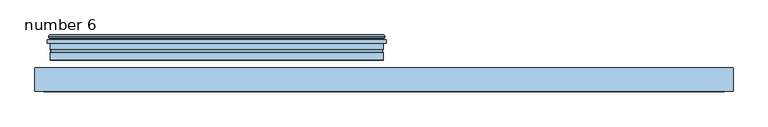
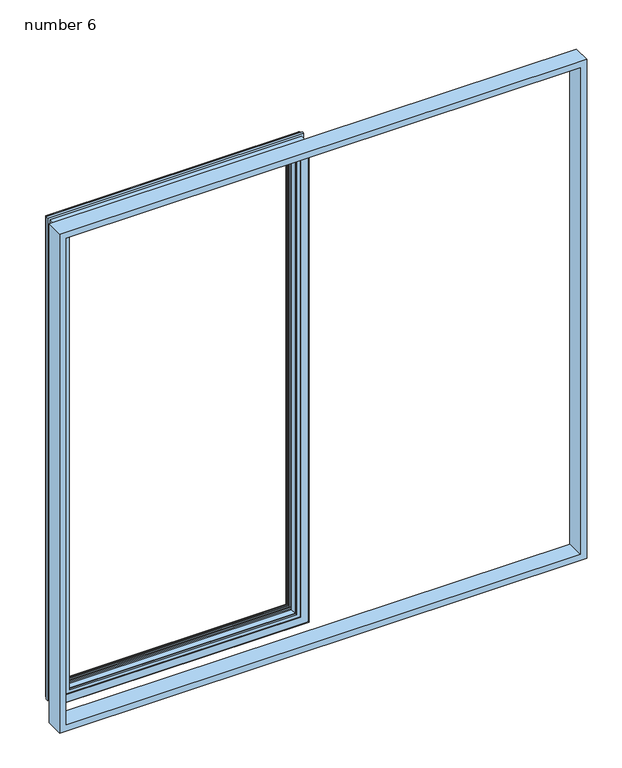
"""IFC4 building model written with IfcOpenShell, lengths in millimetres: window geometry, Window-Exterior-Sierra-Horizontal_Sliding_XO-36inch_Width-Standard : number 6."""

from ifc_helpers import new_model, si_unit, frame, origin, place, context, project, spatial, polyline, ellipse_curve, outline, extrude, source, transform, mapped, element, save
from ifc_brep_helpers import plane_surface, cylinder_surface, revolved_surface, advanced_brep


def number_6_126d4699(model_context):
    return source(origin(), model_context, "Body", "SolidModel", [
        advanced_brep(
        [(-554.92015, 35.099625, 967.49235), (-554.92015, 33.9637671, 967.49235), (-29.27985, 33.9637671, 967.49235), (-29.27985, 35.099625, 967.49235), (-553.0833265, 37.5426644, 969.3291735), (-552.8937762, 35.099625, 969.5187238), (-31.3062238, 35.099625, 969.5187238), (-31.1166735, 37.5426644, 969.3291735), (-560.88915, 40.078025, 961.52335), (-23.31085, 40.078025, 961.52335), (-560.88915, 42.465625, 961.52335), (-23.31085, 42.465625, 961.52335), (-585.57795, 40.078025, 936.83455), (-583.19035, 42.465625, 939.22215), (-1.00965, 42.465625, 939.22215), (1.37795, 40.078025, 936.83455), (-585.57795, 37.512625, 936.83455), (1.37795, 37.512625, 936.83455), (-583.54595, 35.836225, 938.86655), (-583.54595, 37.512625, 938.86655), (-0.65405, 37.512625, 938.86655), (-0.65405, 35.836225, 938.86655), (-580.24395, 33.931225, 942.16855), (-580.24395, 35.836225, 942.16855), (-3.95605, 35.836225, 942.16855), (-3.95605, 33.931225, 942.16855), (-588.16875, 28.317825, 934.24375), (-588.16875, 33.931225, 934.24375), (3.96875, 33.931225, 934.24375), (3.96875, 28.317825, 934.24375), (-582.86015, 16.125825, 939.55235), (-582.86015, 28.317825, 939.55235), (-1.33985, 28.317825, 939.55235), (-1.33985, 16.125825, 939.55235), (-582.86015, 12.163425, 939.55235), (-1.33985, 12.163425, 939.55235), (-582.86015, -1.171575, 939.55235), (-1.33985, -1.171575, 939.55235), (-582.04735, -1.984375, 940.36515), (-2.15265, -1.984375, 940.36515), (-563.75935, -0.103857, 958.65315), (-563.75935, -1.984375, 958.65315), (-20.44065, -1.984375, 958.65315), (-20.44065, -0.103857, 958.65315), (-562.1584612, -1.704057, 960.2540388), (-562.1584612, -0.103857, 960.2540388), (-22.0415388, -0.103857, 960.2540388), (-22.0415388, -1.704057, 960.2540388), (-554.6146612, 2.0638625, 967.7978388), (-554.6146612, -1.704057, 967.7978388), (-29.5853388, -1.704057, 967.7978388), (-29.5853388, 2.0638625, 967.7978388), (-551.4396612, 13.891543, 970.9728388), (-552.4523112, 2.0638625, 969.9601888), (-31.7476888, 2.0638625, 969.9601888), (-32.7603388, 13.891543, 970.9728388), (-563.75935, 11.5032541, 958.65315), (-561.3710612, 13.891543, 961.0414388), (-22.8289388, 13.891543, 961.0414388), (-20.44065, 11.5032541, 958.65315), (-563.75935, 32.940625, 958.65315), (-20.44065, 32.940625, 958.65315), (-559.1555891, 33.9637671, 963.2569109), (-560.1787312, 32.940625, 962.2337688), (-24.0212688, 32.940625, 962.2337688), (-25.0444109, 33.9637671, 963.2569109), (-29.27985, 33.9637671, 2080.50765), (-29.27985, 35.099625, 2080.50765), (-31.3062238, 35.099625, 2078.4812762), (-31.1166735, 37.5426644, 2078.6708265), (-23.31085, 40.078025, 2086.47665), (-23.31085, 42.465625, 2086.47665), (-1.00965, 42.465625, 2108.77785), (1.37795, 40.078025, 2111.16545), (1.37795, 37.512625, 2111.16545), (-0.65405, 37.512625, 2109.13345), (-0.65405, 35.836225, 2109.13345), (-3.95605, 35.836225, 2105.83145), (-3.95605, 33.931225, 2105.83145), (3.96875, 33.931225, 2113.75625), (3.96875, 28.317825, 2113.75625), (-1.33985, 28.317825, 2108.44765), (-1.33985, 16.125825, 2108.44765), (-1.33985, 12.163425, 2108.44765), (-1.33985, -1.171575, 2108.44765), (-2.15265, -1.984375, 2107.63485), (-20.44065, -1.984375, 2089.34685), (-20.44065, -0.103857, 2089.34685), (-22.0415388, -0.103857, 2087.7459612), (-22.0415388, -1.704057, 2087.7459612), (-29.5853388, -1.704057, 2080.2021612), (-29.5853388, 2.0638625, 2080.2021612), (-31.7476888, 2.0638625, 2078.0398112), (-32.7603388, 13.891543, 2077.0271612), (-22.8289388, 13.891543, 2086.9585612), (-20.44065, 11.5032541, 2089.34685), (-20.44065, 32.940625, 2089.34685), (-24.0212688, 32.940625, 2085.7662312), (-25.0444109, 33.9637671, 2084.7430891), (-554.92015, 33.9637671, 2080.50765), (-554.92015, 35.099625, 2080.50765), (-552.8937762, 35.099625, 2078.4812762), (-553.0833265, 37.5426644, 2078.6708265), (-560.88915, 40.078025, 2086.47665), (-560.88915, 42.465625, 2086.47665), (-583.19035, 42.465625, 2108.77785), (-585.57795, 40.078025, 2111.16545), (-585.57795, 37.512625, 2111.16545), (-583.54595, 37.512625, 2109.13345), (-583.54595, 35.836225, 2109.13345), (-580.24395, 35.836225, 2105.83145), (-580.24395, 33.931225, 2105.83145), (-588.16875, 33.931225, 2113.75625), (-588.16875, 28.317825, 2113.75625), (-582.86015, 28.317825, 2108.44765), (-582.86015, 16.125825, 2108.44765), (-582.86015, 12.163425, 2108.44765), (-582.86015, -1.171575, 2108.44765), (-582.04735, -1.984375, 2107.63485), (-563.75935, -1.984375, 2089.34685), (-563.75935, -0.103857, 2089.34685), (-562.1584612, -0.103857, 2087.7459612), (-562.1584612, -1.704057, 2087.7459612), (-554.6146612, -1.704057, 2080.2021612), (-554.6146612, 2.0638625, 2080.2021612), (-552.4523112, 2.0638625, 2078.0398112), (-551.4396612, 13.891543, 2077.0271612), (-561.3710612, 13.891543, 2086.9585612), (-563.75935, 11.5032541, 2089.34685), (-563.75935, 32.940625, 2089.34685), (-560.1787312, 32.940625, 2085.7662312), (-559.1555891, 33.9637671, 2084.7430891)],
        [
            (0, 1),
            (1, 2),
            (2, 3),
            (3, 0),
            (4, 5),
            (5, 6),
            (6, 7),
            (7, 4),
            (8, 4),
            (7, 9),
            (9, 8),
            (10, 8),
            (9, 11),
            (11, 10),
            (12, 13, ellipse_curve(frame((-583.19035, 40.078025, 939.22215), z_axis=(0.7071067811865475, 0.0, -0.7071067811865475), x_axis=(-0.7071067811865476, 0.0, -0.7071067811865474)), 3.3765763, 2.3876)),
            (13, 14),
            (14, 15, ellipse_curve(frame((-1.00965, 40.078025, 939.22215), z_axis=(-0.7071067811865475, 0.0, -0.7071067811865475), x_axis=(-0.7071067811865476, 0.0, 0.7071067811865474)), 3.3765763, 2.3876)),
            (15, 12),
            (16, 12),
            (15, 17),
            (17, 16),
            (18, 19),
            (19, 20),
            (20, 21),
            (21, 18),
            (22, 23),
            (23, 24),
            (24, 25),
            (25, 22),
            (26, 27),
            (27, 28),
            (28, 29),
            (29, 26),
            (30, 31),
            (31, 32),
            (32, 33),
            (33, 30),
            (34, 30, ellipse_curve(frame((-582.86015, 14.144625, 939.55235), z_axis=(-0.7071067811865475, 0.0, 0.7071067811865475), x_axis=(0.7071067811865476, 0.0, 0.7071067811865474)), 2.8018399, 1.9812)),
            (33, 35, ellipse_curve(frame((-1.33985, 14.144625, 939.55235), z_axis=(0.7071067811865475, 0.0, 0.7071067811865475), x_axis=(0.7071067811865476, 0.0, -0.7071067811865474)), 2.8018399, 1.9812)),
            (35, 34),
            (36, 34),
            (35, 37),
            (37, 36),
            (38, 36, ellipse_curve(frame((-582.04735, -1.171575, 940.36515), z_axis=(0.7071067811865475, 0.0, -0.7071067811865475), x_axis=(-0.7071067811865476, 0.0, -0.7071067811865474)), 1.1494728, 0.8128)),
            (37, 39, ellipse_curve(frame((-2.15265, -1.171575, 940.36515), z_axis=(-0.7071067811865475, 0.0, -0.7071067811865475), x_axis=(-0.7071067811865476, 0.0, 0.7071067811865474)), 1.1494728, 0.8128)),
            (39, 38),
            (40, 41),
            (41, 42),
            (42, 43),
            (43, 40),
            (44, 45),
            (45, 46),
            (46, 47),
            (47, 44),
            (48, 49),
            (49, 50),
            (50, 51),
            (51, 48),
            (52, 53),
            (53, 54),
            (54, 55),
            (55, 52),
            (56, 57),
            (57, 58),
            (58, 59),
            (59, 56),
            (60, 56),
            (59, 61),
            (61, 60),
            (62, 63),
            (63, 64),
            (64, 65),
            (65, 62),
            (2, 66),
            (66, 67),
            (67, 3),
            (6, 68),
            (68, 69),
            (69, 7),
            (69, 70),
            (70, 9),
            (70, 71),
            (71, 11),
            (14, 72),
            (72, 73, ellipse_curve(frame((-1.00965, 40.078025, 2108.77785), z_axis=(0.7071067811865475, 0.0, -0.7071067811865475), x_axis=(-0.7071067811865474, 0.0, -0.7071067811865476)), 3.3765763, 2.3876)),
            (73, 15),
            (73, 74),
            (74, 17),
            (20, 75),
            (75, 76),
            (76, 21),
            (24, 77),
            (77, 78),
            (78, 25),
            (28, 79),
            (79, 80),
            (80, 29),
            (32, 81),
            (81, 82),
            (82, 33),
            (82, 83, ellipse_curve(frame((-1.33985, 14.144625, 2108.44765), z_axis=(-0.7071067811865475, 0.0, 0.7071067811865475), x_axis=(0.7071067811865474, 0.0, 0.7071067811865476)), 2.8018399, 1.9812)),
            (83, 35),
            (83, 84),
            (84, 37),
            (84, 85, ellipse_curve(frame((-2.15265, -1.171575, 2107.63485), z_axis=(0.7071067811865475, 0.0, -0.7071067811865475), x_axis=(-0.7071067811865474, 0.0, -0.7071067811865476)), 1.1494728, 0.8128)),
            (85, 39),
            (42, 86),
            (86, 87),
            (87, 43),
            (46, 88),
            (88, 89),
            (89, 47),
            (50, 90),
            (90, 91),
            (91, 51),
            (54, 92),
            (92, 93),
            (93, 55),
            (58, 94),
            (94, 95),
            (95, 59),
            (95, 96),
            (96, 61),
            (64, 97),
            (97, 98),
            (98, 65),
            (66, 99),
            (99, 100),
            (100, 67),
            (68, 101),
            (101, 102),
            (102, 69),
            (102, 103),
            (103, 70),
            (103, 104),
            (104, 71),
            (72, 105),
            (105, 106, ellipse_curve(frame((-583.19035, 40.078025, 2108.77785), z_axis=(0.7071067811865475, 0.0, 0.7071067811865475), x_axis=(0.7071067811865476, 0.0, -0.7071067811865474)), 3.3765763, 2.3876)),
            (106, 73),
            (106, 107),
            (107, 74),
            (75, 108),
            (108, 109),
            (109, 76),
            (77, 110),
            (110, 111),
            (111, 78),
            (79, 112),
            (112, 113),
            (113, 80),
            (81, 114),
            (114, 115),
            (115, 82),
            (115, 116, ellipse_curve(frame((-582.86015, 14.144625, 2108.44765), z_axis=(-0.7071067811865475, 0.0, -0.7071067811865475), x_axis=(-0.7071067811865476, 0.0, 0.7071067811865474)), 2.8018399, 1.9812)),
            (116, 83),
            (116, 117),
            (117, 84),
            (117, 118, ellipse_curve(frame((-582.04735, -1.171575, 2107.63485), z_axis=(0.7071067811865475, 0.0, 0.7071067811865475), x_axis=(0.7071067811865476, 0.0, -0.7071067811865474)), 1.1494728, 0.8128)),
            (118, 85),
            (86, 119),
            (119, 120),
            (120, 87),
            (88, 121),
            (121, 122),
            (122, 89),
            (90, 123),
            (123, 124),
            (124, 91),
            (92, 125),
            (125, 126),
            (126, 93),
            (94, 127),
            (127, 128),
            (128, 95),
            (128, 129),
            (129, 96),
            (97, 130),
            (130, 131),
            (131, 98),
            (131, 62),
            (1, 99),
            (0, 100),
            (5, 101),
            (4, 102),
            (8, 103),
            (10, 104),
            (13, 105),
            (12, 106),
            (16, 107),
            (19, 108),
            (18, 109),
            (23, 110),
            (22, 111),
            (27, 112),
            (26, 113),
            (31, 114),
            (30, 115),
            (34, 116),
            (36, 117),
            (38, 118),
            (41, 119),
            (40, 120),
            (45, 121),
            (44, 122),
            (49, 123),
            (48, 124),
            (53, 125),
            (52, 126),
            (57, 127),
            (56, 128),
            (60, 129),
            (63, 130),
        ],
        [
            plane_surface(frame((-554.92015, 33.9637671, 967.49235), z_axis=(0.0, 0.0, 1.0), x_axis=(1.0, 0.0, 0.0))),
            plane_surface(frame((-552.8937762, 35.099625, 969.5187238), z_axis=(0.0, 0.07735544009934268, 0.9970035786731345), x_axis=(1.0, 0.0, 0.0))),
            plane_surface(frame((-553.0833265, 37.5426644, 969.3291735), z_axis=(0.0, 0.9510889261909005, 0.3089172291683326), x_axis=(1.0, 0.0, 0.0))),
            plane_surface(frame((-560.88915, 40.078025, 961.52335), z_axis=(0.0, 0.0, 1.0), x_axis=(1.0, 0.0, 0.0))),
            cylinder_surface(frame((-588.16875, 40.078025, 939.22215), z_axis=(-1.0, 0.0, 0.0), x_axis=(0.0, -1.0, 0.0)), 2.3876),
            plane_surface(frame((-585.57795, 40.078025, 936.83455), z_axis=(0.0, 0.0, -1.0), x_axis=(1.0, 0.0, 0.0))),
            plane_surface(frame((-583.54595, 37.512625, 938.86655), z_axis=(0.0, 0.0, -1.0), x_axis=(1.0, 0.0, 0.0))),
            plane_surface(frame((-580.24395, 35.836225, 942.16855), z_axis=(0.0, 0.0, -1.0), x_axis=(1.0, 0.0, 0.0))),
            plane_surface(frame((-588.16875, 33.931225, 934.24375), z_axis=(0.0, 0.0, -1.0), x_axis=(1.0, 0.0, 0.0))),
            plane_surface(frame((-582.86015, 28.317825, 939.55235), z_axis=(0.0, 0.0, -1.0), x_axis=(1.0, 0.0, 0.0))),
            revolved_surface(polyline([(0.6413499930890794, 12.163425, 939.55235), (-584.841349993089, 12.163425, 939.55235)]), (-588.16875, 14.144625, 939.55235), (1.0, 0.0, 0.0)),
            plane_surface(frame((-582.86015, 12.163425, 939.55235), z_axis=(0.0, 0.0, -1.0), x_axis=(1.0, 0.0, 0.0))),
            cylinder_surface(frame((-588.16875, -1.171575, 940.36515), z_axis=(-1.0, 0.0, 0.0), x_axis=(0.0, -1.0, 0.0)), 0.8128),
            plane_surface(frame((-563.75935, -1.984375, 958.65315), z_axis=(0.0, 0.0, 1.0), x_axis=(1.0, 0.0, 0.0))),
            plane_surface(frame((-562.1584612, -0.103857, 960.2540388), z_axis=(0.0, 0.0, -1.0), x_axis=(1.0, 0.0, 0.0))),
            plane_surface(frame((-554.6146612, -1.704057, 967.7978388), z_axis=(0.0, 0.0, 1.0), x_axis=(1.0, 0.0, 0.0))),
            plane_surface(frame((-552.4523112, 2.0638625, 969.9601888), z_axis=(0.0, -0.08530487454184647, 0.996354895797376), x_axis=(1.0, 0.0, 0.0))),
            plane_surface(frame((-561.3710612, 13.891543, 961.0414388), z_axis=(0.0, 0.7071067811865713, -0.7071067811865238), x_axis=(1.0, 0.0, 0.0))),
            plane_surface(frame((-563.75935, 11.5032541, 958.65315), z_axis=(0.0, 0.0, 1.0), x_axis=(1.0, 0.0, 0.0))),
            plane_surface(frame((-560.1787312, 32.940625, 962.2337688), z_axis=(0.0, -0.7071067811861558, 0.7071067811869393), x_axis=(1.0, 0.0, 0.0))),
            plane_surface(frame((-29.27985, 33.9637671, 967.49235), z_axis=(-1.0, 0.0, 0.0), x_axis=(0.0, 0.0, 1.0))),
            plane_surface(frame((-31.3062238, 35.099625, 969.5187238), z_axis=(-0.9970035786731345, 0.07735544009934263, 0.0), x_axis=(0.0, 0.0, 1.0))),
            plane_surface(frame((-31.1166735, 37.5426644, 969.3291735), z_axis=(-0.30891722916833264, 0.9510889261909005, 0.0), x_axis=(0.0, 0.0, 1.0))),
            plane_surface(frame((-23.31085, 40.078025, 961.52335), z_axis=(-1.0, 0.0, 0.0), x_axis=(0.0, 0.0, 1.0))),
            cylinder_surface(frame((-1.00965, 40.078025, 934.24375), z_axis=(0.0, 0.0, -1.0), x_axis=(0.0, -1.0, 0.0)), 2.3876),
            plane_surface(frame((1.37795, 40.078025, 936.83455), z_axis=(1.0, 0.0, 0.0), x_axis=(0.0, 0.0, 1.0))),
            plane_surface(frame((-0.65405, 37.512625, 938.86655), z_axis=(1.0, 0.0, 0.0), x_axis=(0.0, 0.0, 1.0))),
            plane_surface(frame((-3.95605, 35.836225, 942.16855), z_axis=(1.0, 0.0, 0.0), x_axis=(0.0, 0.0, 1.0))),
            plane_surface(frame((3.96875, 33.931225, 934.24375), z_axis=(1.0, 0.0, 0.0), x_axis=(0.0, 0.0, 1.0))),
            plane_surface(frame((-1.33985, 28.317825, 939.55235), z_axis=(1.0, 0.0, 0.0), x_axis=(0.0, 0.0, 1.0))),
            revolved_surface(polyline([(-1.33985, 12.163425, 2110.428849993089), (-1.33985, 12.163425, 937.571150006911)]), (-1.33985, 14.144625, 934.24375), (0.0, 0.0, 1.0)),
            plane_surface(frame((-1.33985, 12.163425, 939.55235), z_axis=(1.0, 0.0, 0.0), x_axis=(0.0, 0.0, 1.0))),
            cylinder_surface(frame((-2.15265, -1.171575, 934.24375), z_axis=(0.0, 0.0, -1.0), x_axis=(0.0, -1.0, 0.0)), 0.8128),
            plane_surface(frame((-20.44065, -1.984375, 958.65315), z_axis=(-1.0, 0.0, 0.0), x_axis=(0.0, 0.0, 1.0))),
            plane_surface(frame((-22.0415388, -0.103857, 960.2540388), z_axis=(1.0, 0.0, 0.0), x_axis=(0.0, 0.0, 1.0))),
            plane_surface(frame((-29.5853388, -1.704057, 967.7978388), z_axis=(-1.0, 0.0, 0.0), x_axis=(0.0, 0.0, 1.0))),
            plane_surface(frame((-31.7476888, 2.0638625, 969.9601888), z_axis=(-0.996354895797376, -0.08530487454184653, 0.0), x_axis=(0.0, 0.0, 1.0))),
            plane_surface(frame((-22.8289388, 13.891543, 961.0414388), z_axis=(0.7071067811865238, 0.7071067811865713, 0.0), x_axis=(0.0, 0.0, 1.0))),
            plane_surface(frame((-20.44065, 11.5032541, 958.65315), z_axis=(-1.0, 0.0, 0.0), x_axis=(0.0, 0.0, 1.0))),
            plane_surface(frame((-24.0212688, 32.940625, 962.2337688), z_axis=(-0.7071067811869393, -0.7071067811861558, 0.0), x_axis=(0.0, 0.0, 1.0))),
            plane_surface(frame((-29.27985, 33.9637671, 2080.50765), z_axis=(0.0, 0.0, -1.0), x_axis=(-1.0, 0.0, 0.0))),
            plane_surface(frame((-31.3062238, 35.099625, 2078.4812762), z_axis=(0.0, 0.07735544009934257, -0.9970035786731345), x_axis=(-1.0, 0.0, 0.0))),
            plane_surface(frame((-31.1166735, 37.5426644, 2078.6708265), z_axis=(0.0, 0.9510889261909005, -0.3089172291683327), x_axis=(-1.0, 0.0, 0.0))),
            plane_surface(frame((-23.31085, 40.078025, 2086.47665), z_axis=(0.0, 0.0, -1.0), x_axis=(-1.0, 0.0, 0.0))),
            cylinder_surface(frame((3.96875, 40.078025, 2108.77785), z_axis=(1.0, 0.0, 0.0), x_axis=(0.0, -1.0, 0.0)), 2.3876),
            plane_surface(frame((1.37795, 40.078025, 2111.16545), z_axis=(0.0, 0.0, 1.0), x_axis=(-1.0, 0.0, 0.0))),
            plane_surface(frame((-0.65405, 37.512625, 2109.13345), z_axis=(0.0, 0.0, 1.0), x_axis=(-1.0, 0.0, 0.0))),
            plane_surface(frame((-3.95605, 35.836225, 2105.83145), z_axis=(0.0, 0.0, 1.0), x_axis=(-1.0, 0.0, 0.0))),
            plane_surface(frame((3.96875, 33.931225, 2113.75625), z_axis=(0.0, 0.0, 1.0), x_axis=(-1.0, 0.0, 0.0))),
            plane_surface(frame((-1.33985, 28.317825, 2108.44765), z_axis=(0.0, 0.0, 1.0), x_axis=(-1.0, 0.0, 0.0))),
            revolved_surface(polyline([(-584.841349993089, 12.163425, 2108.44765), (0.6413499930890376, 12.163425, 2108.44765)]), (3.96875, 14.144625, 2108.44765), (-1.0, 0.0, 0.0)),
            plane_surface(frame((-1.33985, 12.163425, 2108.44765), z_axis=(0.0, 0.0, 1.0), x_axis=(-1.0, 0.0, 0.0))),
            cylinder_surface(frame((3.96875, -1.171575, 2107.63485), z_axis=(1.0, 0.0, 0.0), x_axis=(0.0, -1.0, 0.0)), 0.8128),
            plane_surface(frame((-20.44065, -1.984375, 2089.34685), z_axis=(0.0, 0.0, -1.0), x_axis=(-1.0, 0.0, 0.0))),
            plane_surface(frame((-22.0415388, -0.103857, 2087.7459612), z_axis=(0.0, 0.0, 1.0), x_axis=(-1.0, 0.0, 0.0))),
            plane_surface(frame((-29.5853388, -1.704057, 2080.2021612), z_axis=(0.0, 0.0, -1.0), x_axis=(-1.0, 0.0, 0.0))),
            plane_surface(frame((-31.7476888, 2.0638625, 2078.0398112), z_axis=(0.0, -0.08530487454184658, -0.996354895797376), x_axis=(-1.0, 0.0, 0.0))),
            plane_surface(frame((-22.8289388, 13.891543, 2086.9585612), z_axis=(0.0, 0.7071067811865713, 0.7071067811865238), x_axis=(-1.0, 0.0, 0.0))),
            plane_surface(frame((-20.44065, 11.5032541, 2089.34685), z_axis=(0.0, 0.0, -1.0), x_axis=(-1.0, 0.0, 0.0))),
            plane_surface(frame((-24.0212688, 32.940625, 2085.7662312), z_axis=(0.0, -0.7071067811861558, -0.7071067811869393), x_axis=(-1.0, 0.0, 0.0))),
            plane_surface(frame((-559.1555891, 33.9637671, 2084.7430891), z_axis=(0.0, -1.0, 0.0), x_axis=(0.0, 0.0, -1.0))),
            plane_surface(frame((-554.92015, 33.9637671, 2080.50765), z_axis=(1.0, 0.0, 0.0), x_axis=(0.0, 0.0, -1.0))),
            plane_surface(frame((-554.92015, 35.099625, 2080.50765), z_axis=(0.0, -1.0, 0.0), x_axis=(0.0, 0.0, -1.0))),
            plane_surface(frame((-552.8937762, 35.099625, 2078.4812762), z_axis=(0.9970035786731345, 0.07735544009934263, 0.0), x_axis=(0.0, 0.0, -1.0))),
            plane_surface(frame((-553.0833265, 37.5426644, 2078.6708265), z_axis=(0.30891722916833264, 0.9510889261909005, 0.0), x_axis=(0.0, 0.0, -1.0))),
            plane_surface(frame((-560.88915, 40.078025, 2086.47665), z_axis=(1.0, 0.0, 0.0), x_axis=(0.0, 0.0, -1.0))),
            plane_surface(frame((-560.88915, 42.465625, 2086.47665), z_axis=(0.0, 1.0, 0.0), x_axis=(0.0, 0.0, -1.0))),
            cylinder_surface(frame((-583.19035, 40.078025, 2113.75625), z_axis=(0.0, 0.0, 1.0), x_axis=(0.0, -1.0, 0.0)), 2.3876),
            plane_surface(frame((-585.57795, 40.078025, 2111.16545), z_axis=(-1.0, 0.0, 0.0), x_axis=(0.0, 0.0, -1.0))),
            plane_surface(frame((-585.57795, 37.512625, 2111.16545), z_axis=(0.0, -1.0, 0.0), x_axis=(0.0, 0.0, -1.0))),
            plane_surface(frame((-583.54595, 37.512625, 2109.13345), z_axis=(-1.0, 0.0, 0.0), x_axis=(0.0, 0.0, -1.0))),
            plane_surface(frame((-583.54595, 35.836225, 2109.13345), z_axis=(0.0, -1.0, 0.0), x_axis=(0.0, 0.0, -1.0))),
            plane_surface(frame((-580.24395, 35.836225, 2105.83145), z_axis=(-1.0, 0.0, 0.0), x_axis=(0.0, 0.0, -1.0))),
            plane_surface(frame((-580.24395, 33.931225, 2105.83145), z_axis=(0.0, 1.0, 0.0), x_axis=(0.0, 0.0, -1.0))),
            plane_surface(frame((-588.16875, 33.931225, 2113.75625), z_axis=(-1.0, 0.0, 0.0), x_axis=(0.0, 0.0, -1.0))),
            plane_surface(frame((-588.16875, 28.317825, 2113.75625), z_axis=(0.0, -1.0, 0.0), x_axis=(0.0, 0.0, -1.0))),
            plane_surface(frame((-582.86015, 28.317825, 2108.44765), z_axis=(-1.0, 0.0, 0.0), x_axis=(0.0, 0.0, -1.0))),
            revolved_surface(polyline([(-582.86015, 12.163425, 937.5711500069108), (-582.86015, 12.163425, 2110.428849993089)]), (-582.86015, 14.144625, 2113.75625), (0.0, 0.0, -1.0)),
            plane_surface(frame((-582.86015, 12.163425, 2108.44765), z_axis=(-1.0, 0.0, 0.0), x_axis=(0.0, 0.0, -1.0))),
            cylinder_surface(frame((-582.04735, -1.171575, 2113.75625), z_axis=(0.0, 0.0, 1.0), x_axis=(0.0, -1.0, 0.0)), 0.8128),
            plane_surface(frame((-582.04735, -1.984375, 2107.63485), z_axis=(0.0, -1.0, 0.0), x_axis=(0.0, 0.0, -1.0))),
            plane_surface(frame((-563.75935, -1.984375, 2089.34685), z_axis=(1.0, 0.0, 0.0), x_axis=(0.0, 0.0, -1.0))),
            plane_surface(frame((-563.75935, -0.103857, 2089.34685), z_axis=(0.0, -1.0, 0.0), x_axis=(0.0, 0.0, -1.0))),
            plane_surface(frame((-562.1584612, -0.103857, 2087.7459612), z_axis=(-1.0, 0.0, 0.0), x_axis=(0.0, 0.0, -1.0))),
            plane_surface(frame((-562.1584612, -1.704057, 2087.7459612), z_axis=(0.0, -1.0, 0.0), x_axis=(0.0, 0.0, -1.0))),
            plane_surface(frame((-554.6146612, -1.704057, 2080.2021612), z_axis=(1.0, 0.0, 0.0), x_axis=(0.0, 0.0, -1.0))),
            plane_surface(frame((-554.6146612, 2.0638625, 2080.2021612), z_axis=(0.0, -1.0, 0.0), x_axis=(0.0, 0.0, -1.0))),
            plane_surface(frame((-552.4523112, 2.0638625, 2078.0398112), z_axis=(0.996354895797376, -0.08530487454184653, 0.0), x_axis=(0.0, 0.0, -1.0))),
            plane_surface(frame((-551.4396612, 13.891543, 2077.0271612), z_axis=(0.0, 1.0, 0.0), x_axis=(0.0, 0.0, -1.0))),
            plane_surface(frame((-561.3710612, 13.891543, 2086.9585612), z_axis=(-0.7071067811865238, 0.7071067811865713, 0.0), x_axis=(0.0, 0.0, -1.0))),
            plane_surface(frame((-563.75935, 11.5032541, 2089.34685), z_axis=(1.0, 0.0, 0.0), x_axis=(0.0, 0.0, -1.0))),
            plane_surface(frame((-563.75935, 32.940625, 2089.34685), z_axis=(0.0, -1.0, 0.0), x_axis=(0.0, 0.0, -1.0))),
            plane_surface(frame((-560.1787312, 32.940625, 2085.7662312), z_axis=(0.7071067811869393, -0.7071067811861558, 0.0), x_axis=(0.0, 0.0, -1.0))),
        ],
        [
            (0, [[1, 2, 3, 4]]),
            (1, [[5, 6, 7, 8]]),
            (2, [[9, -8, 10, 11]]),
            (3, [[12, -11, 13, 14]]),
            (4, [[15, 16, 17, 18]]),
            (5, [[19, -18, 20, 21]]),
            (6, [[22, 23, 24, 25]]),
            (7, [[26, 27, 28, 29]]),
            (8, [[30, 31, 32, 33]]),
            (9, [[34, 35, 36, 37]]),
            (10, [[38, -37, 39, 40]]),
            (11, [[41, -40, 42, 43]]),
            (12, [[44, -43, 45, 46]]),
            (13, [[47, 48, 49, 50]]),
            (14, [[51, 52, 53, 54]]),
            (15, [[55, 56, 57, 58]]),
            (16, [[59, 60, 61, 62]]),
            (17, [[63, 64, 65, 66]]),
            (18, [[67, -66, 68, 69]]),
            (19, [[70, 71, 72, 73]]),
            (20, [[-3, 74, 75, 76]]),
            (21, [[-7, 77, 78, 79]]),
            (22, [[-10, -79, 80, 81]]),
            (23, [[-13, -81, 82, 83]]),
            (24, [[-17, 84, 85, 86]]),
            (25, [[-20, -86, 87, 88]]),
            (26, [[-24, 89, 90, 91]]),
            (27, [[-28, 92, 93, 94]]),
            (28, [[-32, 95, 96, 97]]),
            (29, [[-36, 98, 99, 100]]),
            (30, [[-39, -100, 101, 102]]),
            (31, [[-42, -102, 103, 104]]),
            (32, [[-45, -104, 105, 106]]),
            (33, [[-49, 107, 108, 109]]),
            (34, [[-53, 110, 111, 112]]),
            (35, [[-57, 113, 114, 115]]),
            (36, [[-61, 116, 117, 118]]),
            (37, [[-65, 119, 120, 121]]),
            (38, [[-68, -121, 122, 123]]),
            (39, [[-72, 124, 125, 126]]),
            (40, [[-75, 127, 128, 129]]),
            (41, [[-78, 130, 131, 132]]),
            (42, [[-80, -132, 133, 134]]),
            (43, [[-82, -134, 135, 136]]),
            (44, [[-85, 137, 138, 139]]),
            (45, [[-87, -139, 140, 141]]),
            (46, [[-90, 142, 143, 144]]),
            (47, [[-93, 145, 146, 147]]),
            (48, [[-96, 148, 149, 150]]),
            (49, [[-99, 151, 152, 153]]),
            (50, [[-101, -153, 154, 155]]),
            (51, [[-103, -155, 156, 157]]),
            (52, [[-105, -157, 158, 159]]),
            (53, [[-108, 160, 161, 162]]),
            (54, [[-111, 163, 164, 165]]),
            (55, [[-114, 166, 167, 168]]),
            (56, [[-117, 169, 170, 171]]),
            (57, [[-120, 172, 173, 174]]),
            (58, [[-122, -174, 175, 176]]),
            (59, [[-125, 177, 178, 179]]),
            (60, [[-126, -179, 180, -73], [181, -127, -74, -2]]),
            (61, [[-128, -181, -1, 182]]),
            (62, [[-76, -129, -182, -4], [183, -130, -77, -6]]),
            (63, [[-131, -183, -5, 184]]),
            (64, [[-133, -184, -9, 185]]),
            (65, [[-135, -185, -12, 186]]),
            (66, [[187, -137, -84, -16], [-83, -136, -186, -14]]),
            (67, [[-138, -187, -15, 188]]),
            (68, [[-140, -188, -19, 189]]),
            (69, [[-88, -141, -189, -21], [190, -142, -89, -23]]),
            (70, [[-143, -190, -22, 191]]),
            (71, [[-91, -144, -191, -25], [192, -145, -92, -27]]),
            (72, [[-146, -192, -26, 193]]),
            (73, [[194, -148, -95, -31], [-94, -147, -193, -29]]),
            (74, [[-149, -194, -30, 195]]),
            (75, [[-97, -150, -195, -33], [196, -151, -98, -35]]),
            (76, [[-152, -196, -34, 197]]),
            (77, [[-154, -197, -38, 198]]),
            (78, [[-156, -198, -41, 199]]),
            (79, [[-158, -199, -44, 200]]),
            (80, [[-106, -159, -200, -46], [201, -160, -107, -48]]),
            (81, [[-161, -201, -47, 202]]),
            (82, [[-109, -162, -202, -50], [203, -163, -110, -52]]),
            (83, [[-164, -203, -51, 204]]),
            (84, [[-112, -165, -204, -54], [205, -166, -113, -56]]),
            (85, [[-167, -205, -55, 206]]),
            (86, [[-115, -168, -206, -58], [207, -169, -116, -60]]),
            (87, [[-170, -207, -59, 208]]),
            (88, [[209, -172, -119, -64], [-118, -171, -208, -62]]),
            (89, [[-173, -209, -63, 210]]),
            (90, [[-175, -210, -67, 211]]),
            (91, [[-123, -176, -211, -69], [212, -177, -124, -71]]),
            (92, [[-178, -212, -70, -180]]),
        ],
    ),
        extrude(outline(polyline([(2133.6, 609.6), (2133.6, -609.6), (914.4, -609.6), (914.4, 609.6), (2133.6, 609.6)]), holes=[polyline([(929.4367932, 594.5632068), (929.4367932, -594.5632068), (2118.5632068, -594.5632068), (2118.5632068, 594.5632068), (929.4367932, 594.5632068)])]), frame((0.0, -56.35625, 0.0), z_axis=(0.0, 1.0, 0.0), x_axis=(0.0, 0.0, 1.0)), (0.0, 0.0, 1.0), 41.7512996),
    ])


if __name__ == "__main__":
    model = new_model("IFC4")
    model_context = context("Model", 3, world=origin())
    ifc_project = project(units=[si_unit("LENGTHUNIT", "METRE", prefix="MILLI")], contexts=[model_context])
    site = spatial("IfcSite", under=ifc_project)
    building = spatial("IfcBuilding", under=site)
    placement = place(None, origin())
    number_6_shape = number_6_126d4699(model_context)
    element("IfcWindow", 1, ObjectType="Window-Exterior-Sierra-Horizontal_Sliding_XO-36inch_Width-Standard : number 6", at=placement, inside=building, context=model_context, shape_type="MappedRepresentation", body=[
        mapped(number_6_shape, transform((0.0, 0.0, 0.0), x_axis=(1.0, 0.0, 0.0), y_axis=(0.0, 1.0, 0.0), z_axis=(0.0, 0.0, 1.0))),
    ])
    save(model, "model.ifc")

# Revit data of these elements
# Type "Window-Exterior-Sierra-Horizontal_Sliding_XO-36inch_Width-Standard : number 6"
#   Type Mark = "54"
#   URL = "http://www.sierrapacificwindows.com"
#   Triple Glaze Note = "Triple glazed options with respective limits"
#   Simulite Note = "Custom Simulite Options Available"
#   Product data url = "https://bimobject.com/sierrapacificwindows/product/sierrapacificwindows_horizontal-sliding-windows"
#   Product Page URL = "http://www.sierrapacificwindows.com/horizontal-sliding-windows.cfm"
#   Product Documentation Link = "http://www.sierrapacificwindows.com/architectural/drawings/pdfs/c-ws_13.pdf"
#   Model = "C-WS-3648"
#   Manufacturer = "Sierra Pacific Windows"
#   Jamb Extension Note = "Extension Jamb may be applied on some applications. Contact your SPW sales rep. for more information"
#   Glass Type = "Insulated Glass"
#   Description = "Energy efficient, durable, and secure window"
#   Construction Type = "Wood/Clad"
#   Assembly Code = "B2030230"
#   Window Pane Thickness = 0' - 0 3/4"
#   Vertical Simulite Length = 3' - 9"
#   Thickness = 0' - 1 3/4"
#   Simulite Wood Thickness Vertical = 0' - 0 11/32"
#   Simulite Wood Thickness Horizontal = 0' - 0 13/32"
#   Simulite Width = 0' - 0 7/8"
#   Simulite Clad Thickness Vertical = 0' - 0 11/32"
#   Simulite Clad Thickness Horizontal = 0' - 0 13/32"
#   Setback = 0' - 0"
#   Rough Width = 5' - 0 3/4"
#   Rough Height = 4' - 0 3/4"
#   Quarter Window Width = 1' - 0 1/2"
#   Interior Setback = 0' - 0"
#   Horizontal Simulite Length = 1' - 9 1/8"
#   Half Frame Width = 2' - 0 7/8"
#   Frame Width = 5' - 0"
#   Height = 4' - 0"
#   Width = 5' - 0"
#   Frame Height = 4' - 0"
#   First Simulite Width = 1' - 8 7/16"
#   First Simulite Height = 3' - 7 9/16"
#   Default Sill Height = 3' - 0"
#   Actual Width = 4' - 0"
#   Actual Height = 4' - 0"
#   Actual Half Width = 2' - 0"
#   Actual Glass Width = 1' - 8 7/16"
#   Actual Glass Height = 3' - 7 9/16"
#   Total Number of Lites Per Panel = 1
#   Simulites Visibility = yes
#   Number of Vertical Simulites Greater than One = 2
#   Number of Vertical Lites Per Panel = 1
#   Number of Horizontal Simulites Greater than One = 2
#   Number of Horizontal Lites Per Panel = 1
#   Vertical Simulite Type = element 483283
#   Interior Simulite = Wood - Sierra Pacific - Pine
#   Interior Panel Material = Wood - Sierra Pacific - Pine
#   Horizontal Simulite Type = element 483288
#   Glass = Glass - Sierra Doors - Clear
#   Frame = douglas fir
#   Exterior Simulite = Paint - Sierra Pacific - White 001
#   Exterior Panel Material = Paint - Sierra Pacific - White 001
#   Wall Closure = (empty or 0)
# Element 1 (IfcWindow, "Window-Exterior-Sierra-Horizontal_Sliding_XO-36inch_Width-Standard : number 6")
#   Materials on its faces: "Wood - Sierra Pacific - Pine", "Paint - Sierra Pacific - White 001", "douglas fir", "Glass - Sierra Doors - Clear"
# Materials
#   "Wood - Sierra Pacific - Pine": class "Miscellaneous", colour RGB 136 105 68, transparency 0
#   "Glass - Sierra Doors - Clear": class "Glass", colour RGB 0 0 255, transparency 0.75
#   "douglas fir": class "Generic", colour RGB 120 120 120, transparency 0, Cost = 0
#   "Paint - Sierra Pacific - White 001": class "Miscellaneous", colour RGB 111 112 111, transparency 0
